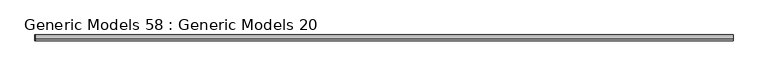
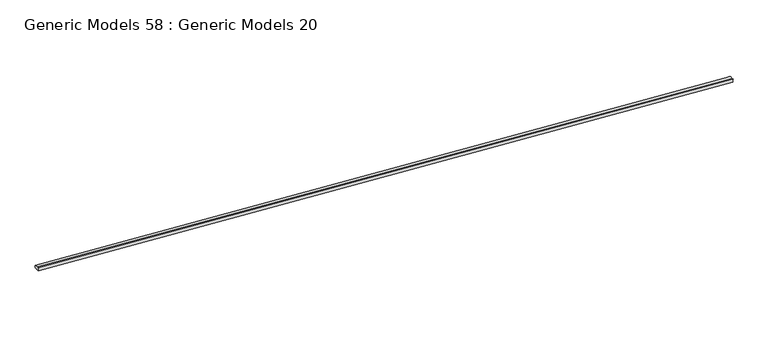
"""IFC4 building model written with IfcOpenShell, lengths in millimetres: proxy geometry, Generic Models 58 : Generic Models 20."""

from ifc_helpers import new_model, si_unit, point, frame, origin, place, context, project, spatial, polyline, circle_curve, ellipse_curve, trimmed, source, transform, mapped, element, save
from ifc_brep_helpers import plane_surface, cylinder_surface, revolved_surface, extruded_surface, advanced_brep


def generic_models_58_generic_models_20_5c2c85ee(model_context):
    return source(origin(), model_context, "Body", "AdvancedBrep", [
        advanced_brep(
        [(27444.1367123, 25523.0152073, 272206.9153252), (27444.5328147, 25523.0152073, 272213.252959), (27444.5328147, 25526.1902073, 272213.252959), (27444.4535532, 25527.1419666, 272211.984775), (27444.2159739, 25527.1419666, 272208.1835092), (27444.1367123, 25526.1902073, 272206.9153252), (28939.8183027, 25523.0152073, 272113.4351647), (28939.8183027, 25526.1902073, 272113.4351647), (28939.8975642, 25527.1419666, 272114.7033488), (28940.1351435, 25527.1419666, 272118.5046145), (28940.214405, 25526.1902073, 272119.7727986), (28940.214405, 25523.0152073, 272119.7727986)],
        [
            (0, 1, circle_curve(frame((27444.3347635, 25520.1004668, 272210.0841421), z_axis=(0.9980525759468362, 0.0, -0.06237832673200686), x_axis=(-0.06237832673200686, 0.0, -0.9980525759468362)), 4.3100275)),
            (1, 2),
            (2, 3, circle_curve(frame((27444.3347635, 25523.2754668, 272210.0841421), z_axis=(-0.9980525759468362, 0.0, 0.06237832673200686), x_axis=(-0.06237832673200686, 0.0, -0.9980525759468362)), 4.3100275)),
            (3, 4, ellipse_curve(frame((27444.3347635, 25530.9527073, 272210.0841421), z_axis=(-0.9980525759468362, 0.0, 0.06237832673200686), x_axis=(0.0, -1.0, 0.0)), 4.7625, 3.175)),
            (4, 5, circle_curve(frame((27444.3347635, 25523.2754668, 272210.0841421), z_axis=(-0.9980525759468362, 0.0, 0.06237832673200686), x_axis=(-0.06237832673200686, 0.0, -0.9980525759468362)), 4.3100275)),
            (5, 0),
            (6, 7),
            (7, 8, circle_curve(frame((28940.0163538, 25523.2754668, 272116.6039817), z_axis=(0.9980525759468362, 0.0, -0.06237832673200686), x_axis=(-0.06237832673200686, 0.0, -0.9980525759468362)), 4.3100275)),
            (8, 9, ellipse_curve(frame((28940.0163538, 25530.9527073, 272116.6039817), z_axis=(0.9980525759468362, 0.0, -0.06237832673200686), x_axis=(0.0, -1.0, 0.0)), 4.7625, 3.175)),
            (9, 10, circle_curve(frame((28940.0163538, 25523.2754668, 272116.6039817), z_axis=(0.9980525759468362, 0.0, -0.06237832673200686), x_axis=(-0.06237832673200686, 0.0, -0.9980525759468362)), 4.3100275)),
            (10, 11),
            (11, 6, circle_curve(frame((28940.0163538, 25520.1004668, 272116.6039817), z_axis=(-0.9980525759468362, 0.0, 0.06237832673200686), x_axis=(-0.06237832673200686, 0.0, -0.9980525759468362)), 4.3100275)),
            (5, 7),
            (6, 0),
            (11, 1),
            (10, 2),
            (9, 3),
            (8, 4),
        ],
        [
            plane_surface(frame((27444.5328147, 25523.0152073, 272213.252959), z_axis=(-0.9980525759468362, 0.0, 0.06237832673200686), x_axis=(0.0, 1.0, 0.0))),
            plane_surface(frame((28940.214405, 25523.0152073, 272119.7727986), z_axis=(0.9980525759468362, 0.0, -0.06237832673200686), x_axis=(0.0, 1.0, 0.0))),
            plane_surface(frame((27444.1367123, 25526.1902073, 272206.9153252), z_axis=(-0.06237832673200577, 0.0, -0.9980525759468362), x_axis=(0.9980525759468362, 0.0, -0.06237832673200577))),
            revolved_surface(polyline([(28939.74750158539, 25520.1004668, 272112.302347606), (27444.065911182024, 25520.1004668, 272205.7825080521)]), (27444.3347635, 25520.1004668, 272210.0841421), (0.9980525759468362, 0.0, -0.06237832673200686)),
            plane_surface(frame((27444.5328147, 25523.0152073, 272213.252959), z_axis=(0.062378326732005954, 0.0, 0.9980525759468362), x_axis=(0.9980525759468362, 0.0, -0.062378326732005954))),
            cylinder_surface(frame((27444.3347635, 25523.2754668, 272210.0841421), z_axis=(-0.9980525759468362, 0.0, 0.06237832673200686), x_axis=(-0.06237832673200686, 0.0, -0.9980525759468362)), 4.3100275),
            extruded_surface(trimmed(ellipse_curve(frame((28940.0163538, 25530.9527073, 272116.6039817), z_axis=(-0.9980525759468362, 0.0, 0.06237832673200686), x_axis=(0.0, -1.0, 0.0)), 4.7625, 3.175), [point((28940.1351435, 25527.1419666, 272118.5046145))], [point((28939.8975642, 25527.1419666, 272114.7033488))], True, "CARTESIAN"), (-1495.6815903000024, 0.0, 93.48016039998038), 1498.5999999835683),
        ],
        [
            (0, [[1, 2, 3, 4, 5, 6]]),
            (1, [[7, 8, 9, 10, 11, 12]]),
            (2, [[-6, 13, -7, 14]]),
            (3, [[-1, -14, -12, 15]]),
            (4, [[-2, -15, -11, 16]]),
            (5, [[-3, -16, -10, 17]]),
            (6, [[-4, -17, -9, 18]]),
            (5, [[-5, -18, -8, -13]]),
        ],
    ),
    ])


if __name__ == "__main__":
    model = new_model("IFC4")
    model_context = context("Model", 3, world=origin())
    ifc_project = project(units=[si_unit("LENGTHUNIT", "METRE", prefix="MILLI")], contexts=[model_context])
    site = spatial("IfcSite", under=ifc_project)
    building = spatial("IfcBuilding", under=site)
    placement = place(None, origin())
    generic_models_58_generic_models_20_shape = generic_models_58_generic_models_20_5c2c85ee(model_context)
    element("IfcBuildingElementProxy", 1, Name="Generic Models 58 : Generic Models 20", ObjectType="Generic Models 58 : Generic Models 20", at=placement, inside=building, context=model_context, shape_type="MappedRepresentation", body=[
        mapped(generic_models_58_generic_models_20_shape, transform((0.0, 0.0, 0.0), x_axis=(1.0, 0.0, 0.0), y_axis=(0.0, 1.0, 0.0), z_axis=(0.0, 0.0, 1.0))),
    ])
    save(model, "model.ifc")

# Revit data of these elements
# Element 1 (IfcBuildingElementProxy, "Generic Models 58 : Generic Models 20")
#   Materials on its faces: "SEALANT (& BACKER ROD IF NECESSARY)"
# Materials
#   "SEALANT (& BACKER ROD IF NECESSARY)": class "Generic", colour RGB 176 213 108, transparency 0, Cost = 0
